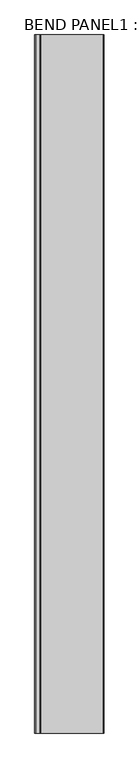
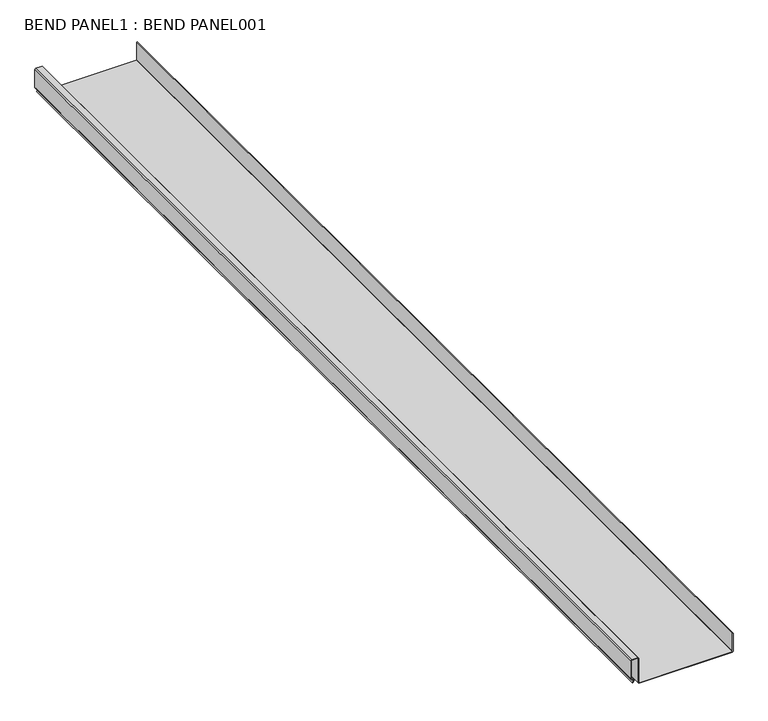
"""IFC4 building model written with IfcOpenShell, lengths in millimetres: proxy geometry, BEND PANEL1 : BEND PANEL001."""

from ifc_helpers import new_model, si_unit, frame, origin, place, context, project, spatial, polyline, outline, extrude, source, transform, mapped, element, save


def bend_panel1_bend_panel001_8c9d74ad(model_context):
    return source(origin(), model_context, "Body", "SweptSolid", [
        extrude(outline(polyline([(42589.7865091, 5848.1043867), (42589.2833292, 5849.1834595), (42594.3520112, 5851.5470247), (42596.210073, 5850.8707455), (42598.2005361, 5846.6022357), (42599.4643694, 5845.8020635), (42634.8859537, 5845.8020635), (42636.2841216, 5847.2002314), (42636.2841216, 5857.8984229), (42634.8859537, 5859.2965908), (42585.9088212, 5859.2965908), (42584.5106533, 5860.6947587), (42584.5106533, 6041.8377287), (42585.9101309, 6043.2372063), (42623.1706509, 6043.2372063), (42623.1706509, 6042.0465813), (42586.4033039, 6042.0465813), (42585.7012783, 6041.3445557), (42585.7012783, 5861.1879317), (42586.4019942, 5860.4872158), (42635.3791267, 5860.4872158), (42637.4747466, 5858.3915959), (42637.4747466, 5846.7070584), (42635.3791267, 5844.6114385), (42599.1191461, 5844.6114385), (42597.268896, 5845.7828894), (42595.3394273, 5849.920598), (42594.4082245, 5850.259528), (42589.7865091, 5848.1043867)])), frame((0.0, -1052.8906574, 0.0), z_axis=(0.0, 1.0, 0.0), x_axis=(0.0, 0.0, 1.0)), (0.0, 0.0, 1.0), 1999.85),
    ])


if __name__ == "__main__":
    model = new_model("IFC4")
    model_context = context("Model", 3, world=origin())
    ifc_project = project(units=[si_unit("LENGTHUNIT", "METRE", prefix="MILLI")], contexts=[model_context])
    site = spatial("IfcSite", under=ifc_project)
    building = spatial("IfcBuilding", under=site)
    placement = place(None, origin())
    bend_panel1_bend_panel001_shape = bend_panel1_bend_panel001_8c9d74ad(model_context)
    element("IfcBuildingElementProxy", 1, Name="BEND PANEL1 : BEND PANEL001", ObjectType="BEND PANEL1 : BEND PANEL001", at=placement, inside=building, context=model_context, shape_type="MappedRepresentation", body=[
        mapped(bend_panel1_bend_panel001_shape, transform((0.0, 0.0, 0.0), x_axis=(1.0, 0.0, 0.0), y_axis=(0.0, 1.0, 0.0), z_axis=(0.0, 0.0, 1.0))),
    ])
    save(model, "model.ifc")

# Revit data of these elements
# Type "BEND PANEL1 : BEND PANEL001"
#   NameOverride = "BEND PANEL001"
# Element 1 (IfcBuildingElementProxy, "BEND PANEL1 : BEND PANEL001")
#   Materials on its faces: "STANDING SEAM METAL ROOF FOLLOW MANU. RECOMMENDED EDGE/TRANSITION DETAILS"
# Materials
#   "STANDING SEAM METAL ROOF FOLLOW MANU. RECOMMENDED EDGE/TRANSITION DETAILS": class "Unassigned", colour RGB 128 128 128, transparency 0, Cost = 0
